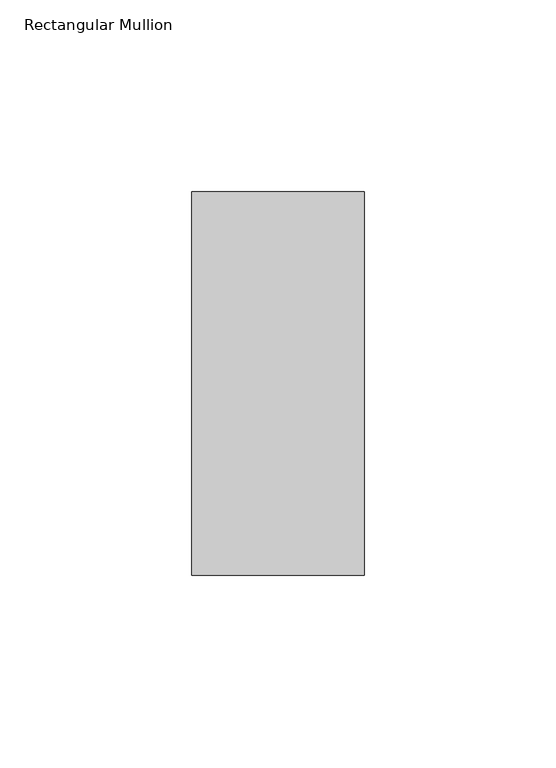
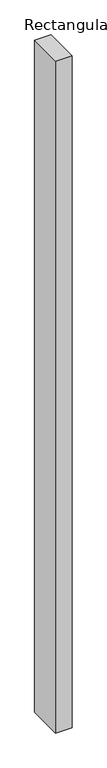
"""IFC4 building model written with IfcOpenShell, lengths in millimetres: member geometry, Rectangular Mullion : 알루미늄_Rectangular Cap_100 x 45."""

from ifc_helpers import new_model, si_unit, frame, origin, place, context, project, spatial, polyline, outline, extrude, source, transform, mapped, element, save


def rectangular_mullion_87973157(model_context):
    return source(origin(), model_context, "Body", "SweptSolid", [
        extrude(outline(polyline([(0.0, 50.0), (0.0, -50.0), (-45.0, -50.0), (-45.0, 50.0), (0.0, 50.0)])), frame((0.0, 0.0, -1961.9999999), z_axis=(0.0, 0.0, 1.0), x_axis=(1.0, 0.0, 0.0)), (0.0, 0.0, 1.0), 1961.9999999),
    ])


if __name__ == "__main__":
    model = new_model("IFC4")
    model_context = context("Model", 3, world=origin())
    ifc_project = project(units=[si_unit("LENGTHUNIT", "METRE", prefix="MILLI")], contexts=[model_context])
    site = spatial("IfcSite", under=ifc_project)
    building = spatial("IfcBuilding", under=site)
    placement = place(None, origin())
    rectangular_mullion_shape = rectangular_mullion_87973157(model_context)
    element("IfcMember", 1, ObjectType="Rectangular Mullion : 알루미늄_Rectangular Cap_100 x 45", at=placement, inside=building, context=model_context, shape_type="MappedRepresentation", body=[
        mapped(rectangular_mullion_shape, transform((0.0, 0.0, 0.0), x_axis=(1.0, 0.0, 0.0), y_axis=(0.0, 1.0, 0.0), z_axis=(0.0, 0.0, 1.0))),
    ])
    save(model, "model.ifc")

# Revit data of these elements
# Type "Rectangular Mullion : 알루미늄_Rectangular Cap_100 x 45"
#   built-in parameter 1007304 = 0.328084 (stored number, unit not read)
#   built-in parameter 1007301 = 0.0738189 (stored number, unit not read)
#   built-in parameter 1007300 = 0.0738189 (stored number, unit not read)
# Element 1 (IfcMember, "Rectangular Mullion : 알루미늄_Rectangular Cap_100 x 45")
#   Materials on its faces: "00_Metal_Stainless Steel"
# Materials
#   "00_Metal_Stainless Steel": class "Metal", colour RGB 148 148 148, transparency 0, Description = "Steel", Cost = 0
